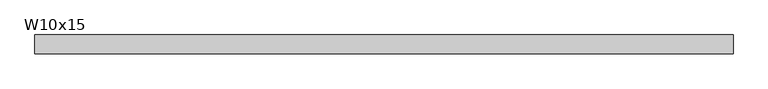
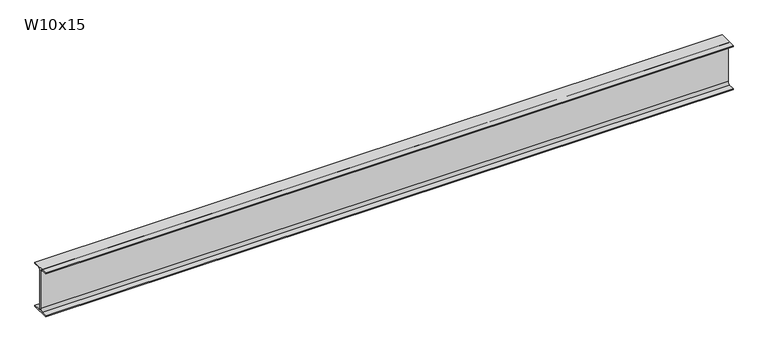
"""IFC4 building model written with IfcOpenShell, lengths in millimetres: beam geometry, RME W-Wide Flange : W10x15."""

import ifcopenshell
import ifcopenshell.guid

model = None  # the IFC model being written
_history = None  # IfcOwnerHistory: only IFC2X3 demands one
_inside = {}  # id of a spatial element -> (the spatial element, [elements in it])
_under = {}  # id of a project, library or spatial element -> (it, [spatial elements below it])
_declared = {}  # id of a project -> (the project, [libraries it declares])
_typed = {}  # id of a type object -> (the type object, [elements of that type])
_made_of = {}  # id of a material, layer set ... -> (it, [elements and type objects made of it])


def new_model(schema):
    """Start an empty IFC model of exactly this schema.

    Asked for "IFC4X3", IfcOpenShell would pick the latest addendum, in which some entities
    have other attributes; the version numbers below select the first issue.
    IFC2X3 requires an IfcOwnerHistory on every rooted entity: one is made here for all.
    """
    global model, _history
    if schema == "IFC4X3":
        model = ifcopenshell.file(schema_version=(4, 3, 0, 0))
    else:
        model = ifcopenshell.file(schema=schema)
    _inside.clear()
    _under.clear()
    _declared.clear()
    _typed.clear()
    _made_of.clear()
    _history = None
    if model.schema == "IFC2X3":
        org = make("IfcOrganization", Name="unknown")
        user = make(
            "IfcPersonAndOrganization",
            ThePerson=make("IfcPerson", FamilyName="unknown"),
            TheOrganization=org,
        )
        app = make(
            "IfcApplication",
            ApplicationDeveloper=org,
            Version="unknown",
            ApplicationFullName="unknown",
            ApplicationIdentifier="unknown",
        )
        _history = make(
            "IfcOwnerHistory",
            OwningUser=user,
            OwningApplication=app,
            ChangeAction="ADDED",
            CreationDate=0,
        )
    return model


def make(cls, **values):
    """One entity of the class cls with the attributes given. An attribute that is None is left unset."""
    return model.create_entity(
        cls, **{name: value for name, value in values.items() if value is not None}
    )


def rooted(cls, **values):
    """An entity with a GlobalId (a new one), such as an element, a storey or a relation."""
    return make(cls, GlobalId=ifcopenshell.guid.new(), OwnerHistory=_history, **values)


def si_unit(unit_type, name, prefix=None):
    """IfcSIUnit, for example si_unit("LENGTHUNIT", "METRE", prefix="MILLI")."""
    return make("IfcSIUnit", UnitType=unit_type, Prefix=prefix, Name=name)


def assignment(units):
    """IfcUnitAssignment: the units of a project."""
    return None if units is None else make("IfcUnitAssignment", Units=units)


def point(xyz):
    """IfcCartesianPoint."""
    return None if xyz is None else make("IfcCartesianPoint", Coordinates=xyz)


def direction(xyz):
    """IfcDirection."""
    return None if xyz is None else make("IfcDirection", DirectionRatios=xyz)


def frame(location, z_axis=None, x_axis=None):
    """IfcAxis2Placement3D, a coordinate frame: its origin and axes. An axis left out is left unset."""
    return make(
        "IfcAxis2Placement3D",
        Location=point(location),
        Axis=direction(z_axis),
        RefDirection=direction(x_axis),
    )


def frame_2d(location, x_axis=None):
    """IfcAxis2Placement2D, a coordinate frame in the plane: its origin and x axis."""
    return make(
        "IfcAxis2Placement2D", Location=point(location), RefDirection=direction(x_axis)
    )


def origin():
    """The frame at (0, 0, 0) with its axes left unset."""
    return frame((0.0, 0.0, 0.0))


def place(relative_to, where):
    """IfcLocalPlacement: puts the frame where relative to a parent placement (None: the world)."""
    return make(
        "IfcLocalPlacement", PlacementRelTo=relative_to, RelativePlacement=where
    )


def context(
    kind, dimensions, precision=None, world=None, true_north=None, identifier=None
):
    """IfcGeometricRepresentationContext, for example the 3D "Model" context."""
    return make(
        "IfcGeometricRepresentationContext",
        ContextIdentifier=identifier,
        ContextType=kind,
        CoordinateSpaceDimension=dimensions,
        Precision=precision,
        WorldCoordinateSystem=world,
        TrueNorth=true_north,
    )


def project(units=None, contexts=None):
    """IfcProject with its units and contexts."""
    return rooted(
        "IfcProject",
        Name="project",
        RepresentationContexts=contexts,
        UnitsInContext=assignment(units),
    )


def spatial(cls, under=None, at=None, **own):
    """A site, building, storey or space (cls), placed at a placement, below another one or the project."""
    s = rooted(cls, ObjectPlacement=at, **own)
    if under is not None:
        _under.setdefault(under.id(), (under, []))[1].append(s)
    return s


def polyline(points):
    """IfcPolyline through the points."""
    return make("IfcPolyline", Points=[point(p) for p in points])


def circle_curve(where, radius):
    """IfcCircle in the frame where."""
    return make("IfcCircle", Position=where, Radius=radius)


def trimmed(basis, trim1, trim2, sense, master):
    """IfcTrimmedCurve: the piece of a basis curve between two trims."""
    return make(
        "IfcTrimmedCurve",
        BasisCurve=basis,
        Trim1=trim1,
        Trim2=trim2,
        SenseAgreement=sense,
        MasterRepresentation=master,
    )


def segment(curve, same_sense, transition):
    """IfcCompositeCurveSegment."""
    return make(
        "IfcCompositeCurveSegment",
        Transition=transition,
        SameSense=same_sense,
        ParentCurve=curve,
    )


def composite_curve(segments, self_intersect=None):
    """IfcCompositeCurve: segments joined end to end."""
    return make("IfcCompositeCurve", Segments=segments, SelfIntersect=self_intersect)


def outline(outer, holes=None, kind="AREA"):
    """IfcArbitraryClosedProfileDef: a profile drawn as a closed curve; with holes, ...WithVoids."""
    if holes is None:
        return make("IfcArbitraryClosedProfileDef", ProfileType=kind, OuterCurve=outer)
    return make(
        "IfcArbitraryProfileDefWithVoids",
        ProfileType=kind,
        OuterCurve=outer,
        InnerCurves=holes,
    )


def extrude(swept, where, along, depth):
    """IfcExtrudedAreaSolid: the profile swept, set in the frame where, extruded along a direction by depth."""
    return make(
        "IfcExtrudedAreaSolid",
        SweptArea=swept,
        Position=where,
        ExtrudedDirection=direction(along),
        Depth=depth,
    )


def shape(context_of_items, identifier, shape_type, items):
    """IfcShapeRepresentation: the items that make up one representation, for example the "Body"."""
    return make(
        "IfcShapeRepresentation",
        ContextOfItems=context_of_items,
        RepresentationIdentifier=identifier,
        RepresentationType=shape_type,
        Items=items,
    )


def source(mapping_origin, context_of_items, identifier, shape_type, items):
    """IfcRepresentationMap: a shape defined once, which mapped items show again and again."""
    return make(
        "IfcRepresentationMap",
        MappingOrigin=mapping_origin,
        MappedRepresentation=shape(context_of_items, identifier, shape_type, items),
    )


def transform(
    local_origin,
    x_axis=None,
    y_axis=None,
    z_axis=None,
    scale=None,
    scale2=None,
    scale3=None,
    uniform=True,
):
    """IfcCartesianTransformationOperator3D, or its non-uniform kind. x_axis, y_axis, z_axis: its Axis1, 2, 3."""
    if uniform:
        return make(
            "IfcCartesianTransformationOperator3D",
            Axis1=direction(x_axis),
            Axis2=direction(y_axis),
            LocalOrigin=point(local_origin),
            Scale=scale,
            Axis3=direction(z_axis),
        )
    return make(
        "IfcCartesianTransformationOperator3DnonUniform",
        Axis1=direction(x_axis),
        Axis2=direction(y_axis),
        LocalOrigin=point(local_origin),
        Scale=scale,
        Axis3=direction(z_axis),
        Scale2=scale2,
        Scale3=scale3,
    )


def mapped(mapping_source, mapping_target):
    """IfcMappedItem: shows the shape of a source again, moved by a transform."""
    return make(
        "IfcMappedItem", MappingSource=mapping_source, MappingTarget=mapping_target
    )


def made_of(thing, what):
    """Note that an element or type object is made of a material, layer set ...; save() writes the relation."""
    if what is not None:
        _made_of.setdefault(what.id(), (what, []))[1].append(thing)
    return thing


def element(
    cls,
    number,
    at=None,
    inside=None,
    cuts=None,
    type_object=None,
    material=None,
    context=None,
    identifier="Body",
    shape_type=None,
    held_by="IfcProductDefinitionShape",
    body=None,
    shapes=None,
    **own,
):
    """One element of the class cls, such as IfcWall. Its Tag is "e" and its number.

    at: its placement. inside: the storey or other place that contains it. cuts: it is an
    opening in that element (IfcRelVoidsElement). A single representation is given by context,
    identifier, shape_type and body (its items); several are given by shapes. held_by: the class
    of the entity that holds the representations. save() writes the other relations.
    """
    e = rooted(cls, Tag="e%d" % number, ObjectPlacement=at, **own)
    if body is not None:
        shapes = [shape(context, identifier, shape_type, body)]
    if shapes is not None:
        e.Representation = make(held_by, Representations=shapes)
    if inside is not None:
        _inside.setdefault(inside.id(), (inside, []))[1].append(e)
    if cuts is not None:
        rooted(
            "IfcRelVoidsElement", RelatingBuildingElement=cuts, RelatedOpeningElement=e
        )
    if type_object is not None:
        _typed.setdefault(type_object.id(), (type_object, []))[1].append(e)
    return made_of(e, material)


def aggregate(whole, parts):
    """IfcRelAggregates: a whole, such as a stair, and the parts it consists of."""
    return rooted("IfcRelAggregates", RelatingObject=whole, RelatedObjects=parts)


def save(model, path):
    """Write the relations noted so far, then the file.

    IfcRelAggregates (storeys below a building ...), IfcRelContainedInSpatialStructure (elements
    in a storey), IfcRelDefinesByType, IfcRelAssociatesMaterial and IfcRelDeclares: one each for
    every whole, place, type object, material and project.
    """
    for whole, parts in _under.values():
        aggregate(whole, parts)
    for where, things in _inside.values():
        rooted(
            "IfcRelContainedInSpatialStructure",
            RelatedElements=things,
            RelatingStructure=where,
        )
    for kind, things in _typed.values():
        rooted("IfcRelDefinesByType", RelatedObjects=things, RelatingType=kind)
    for what, things in _made_of.values():
        rooted("IfcRelAssociatesMaterial", RelatedObjects=things, RelatingMaterial=what)
    for by, libraries in _declared.values():
        rooted("IfcRelDeclares", RelatingContext=by, RelatedDefinitions=libraries)
    model.write(path)


def w10x15_afaa8388(model_context):
    return source(origin(), model_context, "Body", "SweptSolid", [
        extrude(outline(composite_curve([segment(polyline([(50.8, -120.142), (50.8, -127.0), (-50.8, -127.0), (-50.8, -120.142), (-16.7005, -120.142)]), True, "CONTINUOUS"), segment(trimmed(circle_curve(frame_2d((-16.7005, -106.3625)), 13.7795), [point((-16.7005, -120.142))], [point((-2.921, -106.3625))], True, "CARTESIAN"), True, "CONTINUOUS"), segment(polyline([(-2.921, -106.3625), (-2.921, 106.3625)]), True, "CONTINUOUS"), segment(trimmed(circle_curve(frame_2d((-16.7005, 106.3625)), 13.7795), [point((-2.921, 106.3625))], [point((-16.7005, 120.142))], True, "CARTESIAN"), True, "CONTINUOUS"), segment(polyline([(-16.7005, 120.142), (-50.8, 120.142), (-50.8, 127.0), (50.8, 127.0), (50.8, 120.142), (16.7005, 120.142)]), True, "CONTINUOUS"), segment(trimmed(circle_curve(frame_2d((16.7005, 106.3625)), 13.7795), [point((16.7005, 120.142))], [point((2.921, 106.3625))], True, "CARTESIAN"), True, "CONTINUOUS"), segment(polyline([(2.921, 106.3625), (2.921, -106.3625)]), True, "CONTINUOUS"), segment(trimmed(circle_curve(frame_2d((16.7005, -106.3625)), 13.7795), [point((2.921, -106.3625))], [point((16.7005, -120.142))], True, "CARTESIAN"), True, "CONTINUOUS"), segment(polyline([(16.7005, -120.142), (50.8, -120.142)]), True, "CONTINUOUS")], self_intersect=False)), frame((-1866.9, 0.0, 0.0), z_axis=(1.0, 0.0, 0.0), x_axis=(0.0, 1.0, 0.0)), (0.0, 0.0, 1.0), 3733.8),
    ])


if __name__ == "__main__":
    model = new_model("IFC4")
    model_context = context("Model", 3, world=origin())
    ifc_project = project(units=[si_unit("LENGTHUNIT", "METRE", prefix="MILLI")], contexts=[model_context])
    site = spatial("IfcSite", under=ifc_project)
    building = spatial("IfcBuilding", under=site)
    placement = place(None, origin())
    w10x15_shape = w10x15_afaa8388(model_context)
    element("IfcBeam", 1, ObjectType="RME W-Wide Flange : W10x15", at=placement, inside=building, context=model_context, shape_type="MappedRepresentation", body=[
        mapped(w10x15_shape, transform((0.0, 0.0, 0.0), x_axis=(1.0, 0.0, 0.0), y_axis=(0.0, 1.0, 0.0), z_axis=(0.0, 0.0, 1.0))),
    ])
    save(model, "model.ifc")

# Revit data of these elements
# Type "RME W-Wide Flange : W10x15"
#   WELD P [instance default] = ""
#   WELD LE [instance default] = ""
#   WELD D [instance default] = ""
#   TOP SECTION SIZE [instance default] = ""
#   TOP SECTION LENGTH [instance default] = ""
#   REMARKS [instance default] = ""
#   REINF TYPE [instance default] = ""
#   Nominal Size = "W24"
#   End Bearing Capacity [instance default] = ""
#   BOT SECTION SIZE [instance default] = ""
#   BOT SECTION LENGTH [instance default] = ""
#   Assembly Code = "B10"
#   W = 15
#   Start Extension Calculation [instance default] = 10' - 0"
#   Start Extension [instance default] = -0' - 0 1/2"
#   End Extension Calculation [instance default] = 10' - 0"
#   End Extension [instance default] = -0' - 0 1/2"
#   Length [instance default] = 5' - 0"
#   bf = 0' - 4"
#   d = 0' - 10"
#   k = 0' - 0 13/16"
#   k2 = 0' - 0.5425"
#   tf = 0' - 0.27"
#   tw = 0' - 0.23"
#   A = 0.030625 SF
#   Structural Material [instance default] = Metal - Steel - ASTM A992
# Element 1 (IfcBeam, "RME W-Wide Flange : W10x15")
#   Length = 12' - 3"
#   Materials on its faces: "Metal - Steel - ASTM A992"
# Materials
#   "Metal - Steel - ASTM A992": class "Metal", colour RGB 255 128 0, transparency 0
